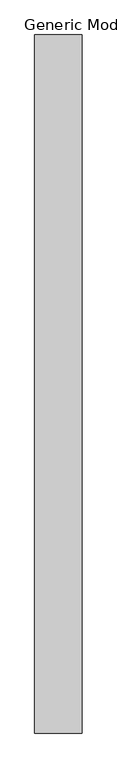
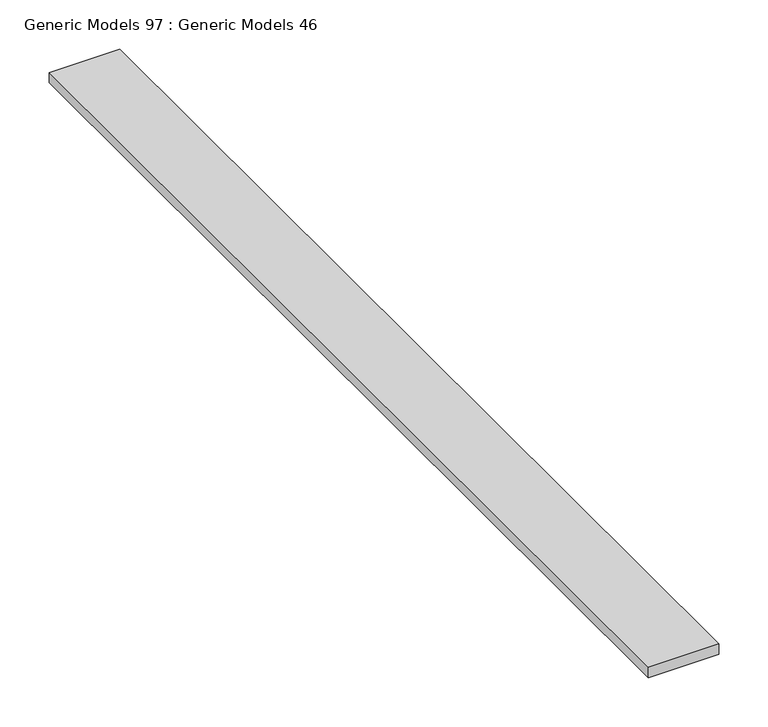
"""IFC4 building model written with IfcOpenShell, lengths in millimetres: proxy geometry, Generic Models 97 : Generic Models 46."""

import ifcopenshell
import ifcopenshell.guid

model = None  # the IFC model being written
_history = None  # IfcOwnerHistory: only IFC2X3 demands one
_inside = {}  # id of a spatial element -> (the spatial element, [elements in it])
_under = {}  # id of a project, library or spatial element -> (it, [spatial elements below it])
_declared = {}  # id of a project -> (the project, [libraries it declares])
_typed = {}  # id of a type object -> (the type object, [elements of that type])
_made_of = {}  # id of a material, layer set ... -> (it, [elements and type objects made of it])


def new_model(schema):
    """Start an empty IFC model of exactly this schema.

    Asked for "IFC4X3", IfcOpenShell would pick the latest addendum, in which some entities
    have other attributes; the version numbers below select the first issue.
    IFC2X3 requires an IfcOwnerHistory on every rooted entity: one is made here for all.
    """
    global model, _history
    if schema == "IFC4X3":
        model = ifcopenshell.file(schema_version=(4, 3, 0, 0))
    else:
        model = ifcopenshell.file(schema=schema)
    _inside.clear()
    _under.clear()
    _declared.clear()
    _typed.clear()
    _made_of.clear()
    _history = None
    if model.schema == "IFC2X3":
        org = make("IfcOrganization", Name="unknown")
        user = make(
            "IfcPersonAndOrganization",
            ThePerson=make("IfcPerson", FamilyName="unknown"),
            TheOrganization=org,
        )
        app = make(
            "IfcApplication",
            ApplicationDeveloper=org,
            Version="unknown",
            ApplicationFullName="unknown",
            ApplicationIdentifier="unknown",
        )
        _history = make(
            "IfcOwnerHistory",
            OwningUser=user,
            OwningApplication=app,
            ChangeAction="ADDED",
            CreationDate=0,
        )
    return model


def make(cls, **values):
    """One entity of the class cls with the attributes given. An attribute that is None is left unset."""
    return model.create_entity(
        cls, **{name: value for name, value in values.items() if value is not None}
    )


def rooted(cls, **values):
    """An entity with a GlobalId (a new one), such as an element, a storey or a relation."""
    return make(cls, GlobalId=ifcopenshell.guid.new(), OwnerHistory=_history, **values)


def si_unit(unit_type, name, prefix=None):
    """IfcSIUnit, for example si_unit("LENGTHUNIT", "METRE", prefix="MILLI")."""
    return make("IfcSIUnit", UnitType=unit_type, Prefix=prefix, Name=name)


def assignment(units):
    """IfcUnitAssignment: the units of a project."""
    return None if units is None else make("IfcUnitAssignment", Units=units)


def point(xyz):
    """IfcCartesianPoint."""
    return None if xyz is None else make("IfcCartesianPoint", Coordinates=xyz)


def direction(xyz):
    """IfcDirection."""
    return None if xyz is None else make("IfcDirection", DirectionRatios=xyz)


def frame(location, z_axis=None, x_axis=None):
    """IfcAxis2Placement3D, a coordinate frame: its origin and axes. An axis left out is left unset."""
    return make(
        "IfcAxis2Placement3D",
        Location=point(location),
        Axis=direction(z_axis),
        RefDirection=direction(x_axis),
    )


def origin():
    """The frame at (0, 0, 0) with its axes left unset."""
    return frame((0.0, 0.0, 0.0))


def place(relative_to, where):
    """IfcLocalPlacement: puts the frame where relative to a parent placement (None: the world)."""
    return make(
        "IfcLocalPlacement", PlacementRelTo=relative_to, RelativePlacement=where
    )


def context(
    kind, dimensions, precision=None, world=None, true_north=None, identifier=None
):
    """IfcGeometricRepresentationContext, for example the 3D "Model" context."""
    return make(
        "IfcGeometricRepresentationContext",
        ContextIdentifier=identifier,
        ContextType=kind,
        CoordinateSpaceDimension=dimensions,
        Precision=precision,
        WorldCoordinateSystem=world,
        TrueNorth=true_north,
    )


def project(units=None, contexts=None):
    """IfcProject with its units and contexts."""
    return rooted(
        "IfcProject",
        Name="project",
        RepresentationContexts=contexts,
        UnitsInContext=assignment(units),
    )


def spatial(cls, under=None, at=None, **own):
    """A site, building, storey or space (cls), placed at a placement, below another one or the project."""
    s = rooted(cls, ObjectPlacement=at, **own)
    if under is not None:
        _under.setdefault(under.id(), (under, []))[1].append(s)
    return s


def polyline(points):
    """IfcPolyline through the points."""
    return make("IfcPolyline", Points=[point(p) for p in points])


def outline(outer, holes=None, kind="AREA"):
    """IfcArbitraryClosedProfileDef: a profile drawn as a closed curve; with holes, ...WithVoids."""
    if holes is None:
        return make("IfcArbitraryClosedProfileDef", ProfileType=kind, OuterCurve=outer)
    return make(
        "IfcArbitraryProfileDefWithVoids",
        ProfileType=kind,
        OuterCurve=outer,
        InnerCurves=holes,
    )


def extrude(swept, where, along, depth):
    """IfcExtrudedAreaSolid: the profile swept, set in the frame where, extruded along a direction by depth."""
    return make(
        "IfcExtrudedAreaSolid",
        SweptArea=swept,
        Position=where,
        ExtrudedDirection=direction(along),
        Depth=depth,
    )


def shape(context_of_items, identifier, shape_type, items):
    """IfcShapeRepresentation: the items that make up one representation, for example the "Body"."""
    return make(
        "IfcShapeRepresentation",
        ContextOfItems=context_of_items,
        RepresentationIdentifier=identifier,
        RepresentationType=shape_type,
        Items=items,
    )


def source(mapping_origin, context_of_items, identifier, shape_type, items):
    """IfcRepresentationMap: a shape defined once, which mapped items show again and again."""
    return make(
        "IfcRepresentationMap",
        MappingOrigin=mapping_origin,
        MappedRepresentation=shape(context_of_items, identifier, shape_type, items),
    )


def transform(
    local_origin,
    x_axis=None,
    y_axis=None,
    z_axis=None,
    scale=None,
    scale2=None,
    scale3=None,
    uniform=True,
):
    """IfcCartesianTransformationOperator3D, or its non-uniform kind. x_axis, y_axis, z_axis: its Axis1, 2, 3."""
    if uniform:
        return make(
            "IfcCartesianTransformationOperator3D",
            Axis1=direction(x_axis),
            Axis2=direction(y_axis),
            LocalOrigin=point(local_origin),
            Scale=scale,
            Axis3=direction(z_axis),
        )
    return make(
        "IfcCartesianTransformationOperator3DnonUniform",
        Axis1=direction(x_axis),
        Axis2=direction(y_axis),
        LocalOrigin=point(local_origin),
        Scale=scale,
        Axis3=direction(z_axis),
        Scale2=scale2,
        Scale3=scale3,
    )


def mapped(mapping_source, mapping_target):
    """IfcMappedItem: shows the shape of a source again, moved by a transform."""
    return make(
        "IfcMappedItem", MappingSource=mapping_source, MappingTarget=mapping_target
    )


def made_of(thing, what):
    """Note that an element or type object is made of a material, layer set ...; save() writes the relation."""
    if what is not None:
        _made_of.setdefault(what.id(), (what, []))[1].append(thing)
    return thing


def element(
    cls,
    number,
    at=None,
    inside=None,
    cuts=None,
    type_object=None,
    material=None,
    context=None,
    identifier="Body",
    shape_type=None,
    held_by="IfcProductDefinitionShape",
    body=None,
    shapes=None,
    **own,
):
    """One element of the class cls, such as IfcWall. Its Tag is "e" and its number.

    at: its placement. inside: the storey or other place that contains it. cuts: it is an
    opening in that element (IfcRelVoidsElement). A single representation is given by context,
    identifier, shape_type and body (its items); several are given by shapes. held_by: the class
    of the entity that holds the representations. save() writes the other relations.
    """
    e = rooted(cls, Tag="e%d" % number, ObjectPlacement=at, **own)
    if body is not None:
        shapes = [shape(context, identifier, shape_type, body)]
    if shapes is not None:
        e.Representation = make(held_by, Representations=shapes)
    if inside is not None:
        _inside.setdefault(inside.id(), (inside, []))[1].append(e)
    if cuts is not None:
        rooted(
            "IfcRelVoidsElement", RelatingBuildingElement=cuts, RelatedOpeningElement=e
        )
    if type_object is not None:
        _typed.setdefault(type_object.id(), (type_object, []))[1].append(e)
    return made_of(e, material)


def aggregate(whole, parts):
    """IfcRelAggregates: a whole, such as a stair, and the parts it consists of."""
    return rooted("IfcRelAggregates", RelatingObject=whole, RelatedObjects=parts)


def save(model, path):
    """Write the relations noted so far, then the file.

    IfcRelAggregates (storeys below a building ...), IfcRelContainedInSpatialStructure (elements
    in a storey), IfcRelDefinesByType, IfcRelAssociatesMaterial and IfcRelDeclares: one each for
    every whole, place, type object, material and project.
    """
    for whole, parts in _under.values():
        aggregate(whole, parts)
    for where, things in _inside.values():
        rooted(
            "IfcRelContainedInSpatialStructure",
            RelatedElements=things,
            RelatingStructure=where,
        )
    for kind, things in _typed.values():
        rooted("IfcRelDefinesByType", RelatedObjects=things, RelatingType=kind)
    for what, things in _made_of.values():
        rooted("IfcRelAssociatesMaterial", RelatedObjects=things, RelatingMaterial=what)
    for by, libraries in _declared.values():
        rooted("IfcRelDeclares", RelatingContext=by, RelatedDefinitions=libraries)
    model.write(path)


def generic_models_97_generic_models_46_9b58c67a(model_context):
    return source(origin(), model_context, "Body", "SweptSolid", [
        extrude(outline(polyline([(48150.8590144, 0.0), (48067.9695022, 0.0), (48067.9695022, 1219.2), (48150.8590144, 1219.2), (48150.8590144, 0.0)])), frame((0.0, 0.0, 999.573933), z_axis=(0.0, 0.0, 1.0), x_axis=(1.0, 0.0, 0.0)), (0.0, 0.0, 1.0), 12.8984375),
    ])


if __name__ == "__main__":
    model = new_model("IFC4")
    model_context = context("Model", 3, world=origin())
    ifc_project = project(units=[si_unit("LENGTHUNIT", "METRE", prefix="MILLI")], contexts=[model_context])
    site = spatial("IfcSite", under=ifc_project)
    building = spatial("IfcBuilding", under=site)
    placement = place(None, origin())
    generic_models_97_generic_models_46_shape = generic_models_97_generic_models_46_9b58c67a(model_context)
    element("IfcBuildingElementProxy", 1, Name="Generic Models 97 : Generic Models 46", ObjectType="Generic Models 97 : Generic Models 46", at=placement, inside=building, context=model_context, shape_type="MappedRepresentation", body=[
        mapped(generic_models_97_generic_models_46_shape, transform((0.0, 0.0, 0.0), x_axis=(1.0, 0.0, 0.0), y_axis=(0.0, 1.0, 0.0), z_axis=(0.0, 0.0, 1.0))),
    ])
    save(model, "model.ifc")

# Revit data of these elements
# Element 1 (IfcBuildingElementProxy, "Generic Models 97 : Generic Models 46")
#   Materials on its faces: "BLOCKING - SIZE AS NEC."
# Materials
#   "BLOCKING - SIZE AS NEC.": class "Wood", colour RGB 234 198 147, transparency 0, Description = "Pinus Echinata", Cost = 0
